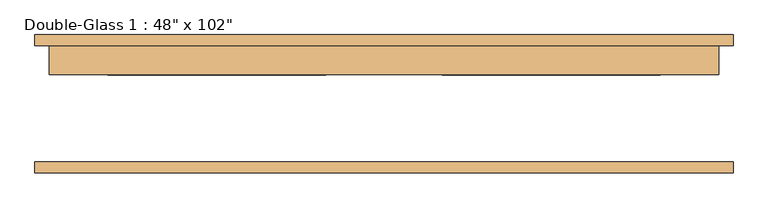
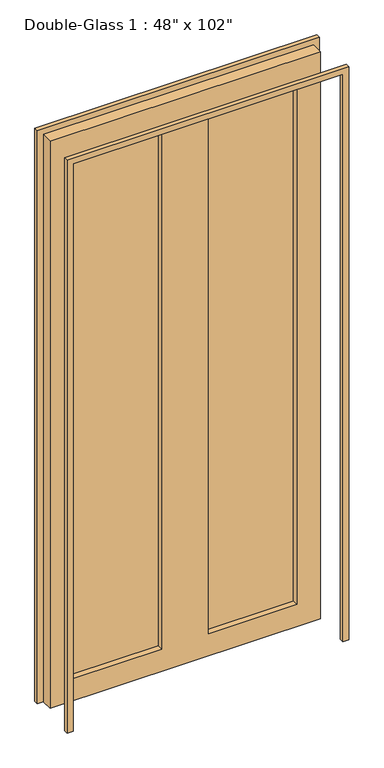
"""IFC4 building model written with IfcOpenShell, lengths in millimetres: door geometry."""

from ifc_helpers import new_model, si_unit, frame, origin, place, context, project, spatial, polyline, outline, extrude, source, transform, mapped, element, save


def door_c2aae917(model_context):
    return source(origin(), model_context, "Body", "SweptSolid", [
        extrude(outline(polyline([(0.0, 609.6), (2616.2, 609.6), (2616.2, -609.6), (0.0, -609.6), (0.0, -584.2), (2590.8, -584.2), (2590.8, 584.2), (0.0, 584.2), (0.0, 609.6)])), frame((0.0, -118.26875, 0.0), z_axis=(0.0, 1.0, 0.0), x_axis=(0.0, 0.0, 1.0)), (0.0, 0.0, 1.0), 19.05),
        extrude(outline(polyline([(2590.8, 584.2), (0.0, 584.2), (0.0, 609.6), (2616.2, 609.6), (2616.2, -609.6), (0.0, -609.6), (0.0, -584.2), (2590.8, -584.2), (2590.8, 584.2)])), frame((0.0, 103.98125, 0.0), z_axis=(0.0, 1.0, 0.0), x_axis=(0.0, 0.0, 1.0)), (0.0, 0.0, 1.0), 19.05),
        extrude(outline(polyline([(482.6, 78.58125), (101.6, 78.58125), (101.6, 85.725), (482.6, 85.725), (482.6, 78.58125)])), frame((0.0, 0.0, 101.6), z_axis=(0.0, 0.0, 1.0), x_axis=(1.0, 0.0, 0.0)), (0.0, 0.0, 1.0), 2387.6),
        extrude(outline(polyline([(-101.6, 78.58125), (-482.6, 78.58125), (-482.6, 85.725), (-101.6, 85.725), (-101.6, 78.58125)])), frame((0.0, 0.0, 101.6), z_axis=(0.0, 0.0, 1.0), x_axis=(1.0, 0.0, 0.0)), (0.0, 0.0, 1.0), 2387.6),
        extrude(outline(polyline([(2590.8, 584.2), (2590.8, -584.2), (0.0, -584.2), (0.0, 584.2), (2590.8, 584.2)]), holes=[polyline([(2489.2, -101.6), (101.6, -101.6), (101.6, -482.6), (2489.2, -482.6), (2489.2, -101.6)]), polyline([(2489.2, 482.6), (101.6, 482.6), (101.6, 101.6), (2489.2, 101.6), (2489.2, 482.6)])]), frame((0.0, 53.18125, 0.0), z_axis=(0.0, 1.0, 0.0), x_axis=(0.0, 0.0, 1.0)), (0.0, 0.0, 1.0), 50.8),
    ])


if __name__ == "__main__":
    model = new_model("IFC4")
    model_context = context("Model", 3, world=origin())
    ifc_project = project(units=[si_unit("LENGTHUNIT", "METRE", prefix="MILLI")], contexts=[model_context])
    site = spatial("IfcSite", under=ifc_project)
    building = spatial("IfcBuilding", under=site)
    placement = place(None, origin())
    door_shape = door_c2aae917(model_context)
    element("IfcDoor", 1, ObjectType="Double-Glass 1 : 48\" x 102\"", at=placement, inside=building, context=model_context, shape_type="MappedRepresentation", body=[
        mapped(door_shape, transform((0.0, 0.0, 0.0), x_axis=(1.0, 0.0, 0.0), y_axis=(0.0, 1.0, 0.0), z_axis=(0.0, 0.0, 1.0))),
    ])
    save(model, "model.ifc")

# Revit data of these elements
# Type "Double-Glass 1 : 48\" x 102\""
#   Type Mark = "30"
#   Assembly Code = "C1020"
#   Thickness = 0' - 2"
#   Height = 8' - 6"
#   Rail Width - Base = 0' - 4"
#   Rail Width - Top = 0' - 4"
#   Stile Width - Hinge = 0' - 4"
#   Stile Width - Latch = 0' - 4"
#   Trim Projection = 0' - 0 3/4"
#   Trim Width = 0' - 1"
#   Width = 3' - 10"
#   Door Material = Door - Panel
#   Frame Material = Door - Frame
#   Function = (empty or 0)
#   Wall Closure = (empty or 0)
# Element 1 (IfcDoor, "Double-Glass 1 : 48\" x 102\"")
#   Materials on its faces: "Door - Frame", "Door - Panel", "Glass"
# Materials
#   "Door - Panel": class "Wood", colour RGB 210 159 95, transparency 0
#   "Door - Frame": class "Miscellaneous", colour RGB 118 70 51, transparency 0
#   "Glass": class "Glass", colour RGB 0 128 192, transparency 0.75
